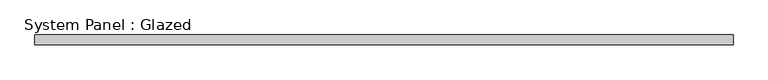
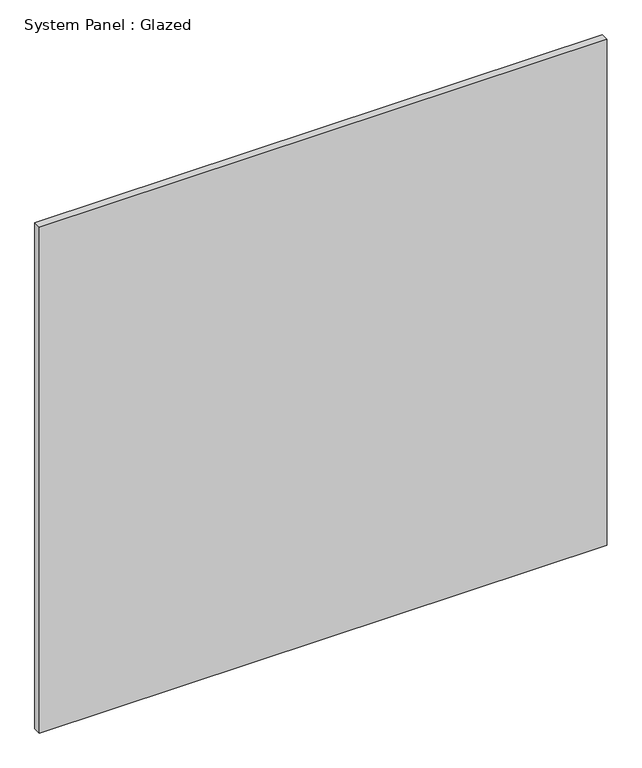
"""IFC4 building model written with IfcOpenShell, lengths in millimetres: plate geometry, System Panel : Glazed."""

from ifc_helpers import new_model, si_unit, origin, origin_with_axes, place, context, project, spatial, polyline, outline, extrude, source, transform, mapped, element, save


def system_panel_glazed_a325710e(model_context):
    return source(origin(), model_context, "Body", "SweptSolid", [
        extrude(outline(polyline([(902.5000002, 24.5), (-902.5000002, 24.5), (-902.5000002, 49.5), (902.5000002, 49.5), (902.5000002, 24.5)])), origin_with_axes(), (0.0, 0.0, 1.0), 1699.4222628),
    ])


if __name__ == "__main__":
    model = new_model("IFC4")
    model_context = context("Model", 3, world=origin())
    ifc_project = project(units=[si_unit("LENGTHUNIT", "METRE", prefix="MILLI")], contexts=[model_context])
    site = spatial("IfcSite", under=ifc_project)
    building = spatial("IfcBuilding", under=site)
    placement = place(None, origin())
    system_panel_glazed_shape = system_panel_glazed_a325710e(model_context)
    element("IfcPlate", 1, ObjectType="System Panel : Glazed", at=placement, inside=building, context=model_context, shape_type="MappedRepresentation", body=[
        mapped(system_panel_glazed_shape, transform((0.0, 0.0, 0.0), x_axis=(1.0, 0.0, 0.0), y_axis=(0.0, 1.0, 0.0), z_axis=(0.0, 0.0, 1.0))),
    ])
    save(model, "model.ifc")

# Revit data of these elements
# Element 1 (IfcPlate, "System Panel : Glazed")
#   Materials on its faces: "Glass"
# Materials
#   "Glass": class "Glass", colour RGB 218 227 224, transparency 0.85, Description = "Soda Lime Glass", Cost = 0
